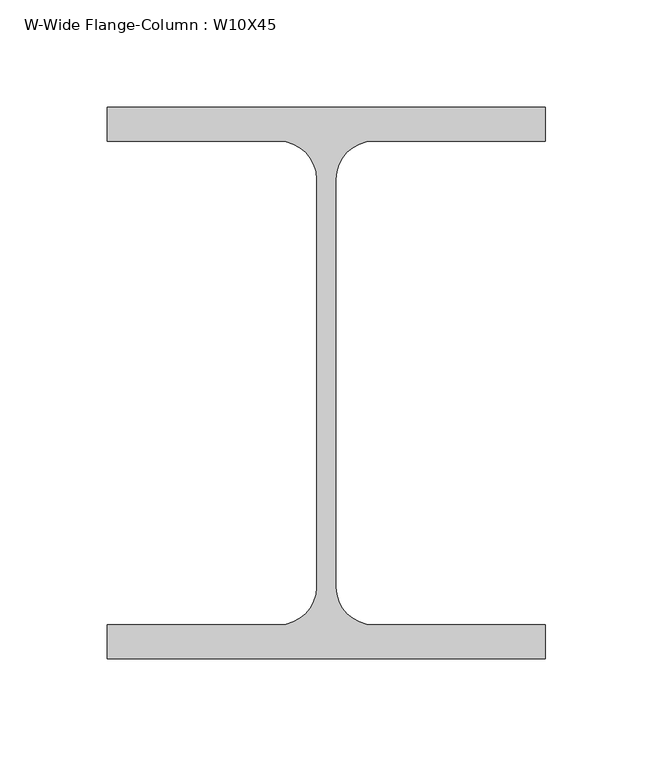
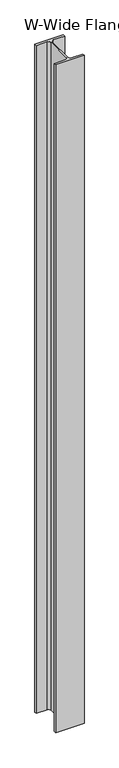
"""IFC4 building model written with IfcOpenShell, lengths in millimetres: column geometry, W-Wide Flange-Column : W10X45."""

from ifc_helpers import new_model, si_unit, point, frame, frame_2d, origin, place, context, project, spatial, polyline, circle_curve, trimmed, segment, composite_curve, outline, extrude, source, transform, mapped, element, save


def w_wide_flange_column_w10x45_583dc8cf(model_context):
    return source(origin(), model_context, "Body", "SweptSolid", [
        extrude(outline(composite_curve([segment(polyline([(101.854, 128.27), (101.854, 112.522), (22.0345, 112.522)]), True, "CONTINUOUS"), segment(trimmed(circle_curve(frame_2d((22.0345, 94.9325)), 17.5895), [point((22.0345, 112.522))], [point((4.445, 94.9325))], True, "CARTESIAN"), True, "CONTINUOUS"), segment(polyline([(4.445, 94.9325), (4.445, -94.9325)]), True, "CONTINUOUS"), segment(trimmed(circle_curve(frame_2d((22.0345, -94.9325)), 17.5895), [point((4.445, -94.9325))], [point((22.0345, -112.522))], True, "CARTESIAN"), True, "CONTINUOUS"), segment(polyline([(22.0345, -112.522), (101.854, -112.522), (101.854, -128.27), (-101.854, -128.27), (-101.854, -112.522), (-22.0345, -112.522)]), True, "CONTINUOUS"), segment(trimmed(circle_curve(frame_2d((-22.0345, -94.9325)), 17.5895), [point((-22.0345, -112.522))], [point((-4.445, -94.9325))], True, "CARTESIAN"), True, "CONTINUOUS"), segment(polyline([(-4.445, -94.9325), (-4.445, 94.9325)]), True, "CONTINUOUS"), segment(trimmed(circle_curve(frame_2d((-22.0345, 94.9325)), 17.5895), [point((-4.445, 94.9325))], [point((-22.0345, 112.522))], True, "CARTESIAN"), True, "CONTINUOUS"), segment(polyline([(-22.0345, 112.522), (-101.854, 112.522), (-101.854, 128.27), (101.854, 128.27)]), True, "CONTINUOUS")], self_intersect=False)), frame((0.0, 0.0, 12566.65), z_axis=(0.0, 0.0, 1.0), x_axis=(1.0, 0.0, 0.0)), (0.0, 0.0, 1.0), 5060.95),
    ])


if __name__ == "__main__":
    model = new_model("IFC4")
    model_context = context("Model", 3, world=origin())
    ifc_project = project(units=[si_unit("LENGTHUNIT", "METRE", prefix="MILLI")], contexts=[model_context])
    site = spatial("IfcSite", under=ifc_project)
    building = spatial("IfcBuilding", under=site)
    placement = place(None, origin())
    w_wide_flange_column_w10x45_shape = w_wide_flange_column_w10x45_583dc8cf(model_context)
    element("IfcColumn", 1, ObjectType="W-Wide Flange-Column : W10X45", at=placement, inside=building, context=model_context, shape_type="MappedRepresentation", body=[
        mapped(w_wide_flange_column_w10x45_shape, transform((0.0, 0.0, 0.0), x_axis=(1.0, 0.0, 0.0), y_axis=(0.0, 1.0, 0.0), z_axis=(0.0, 0.0, 1.0))),
    ])
    save(model, "model.ifc")

# Revit data of these elements
# Type "W-Wide Flange-Column : W10X45"
#   Assembly Code = "B10"
#   W = 45
#   bf = 0' - 8.02"
#   d = 0' - 10.1"
#   k = 0' - 1 5/16"
#   kr = 0' - 0.6925"
#   tf = 0' - 0.62"
#   tw = 0' - 0.35"
#   A = 0.0923611 SF
#   Structural Material [instance default] = Steel ASTM A992
# Element 1 (IfcColumn, "W-Wide Flange-Column : W10X45")
#   Materials on its faces: "Steel ASTM A992"
# Materials
#   "Steel ASTM A992": class "Metal", colour RGB 199 199 199, transparency 0, Description = "Structural steel 50ksi", Cost = 0
